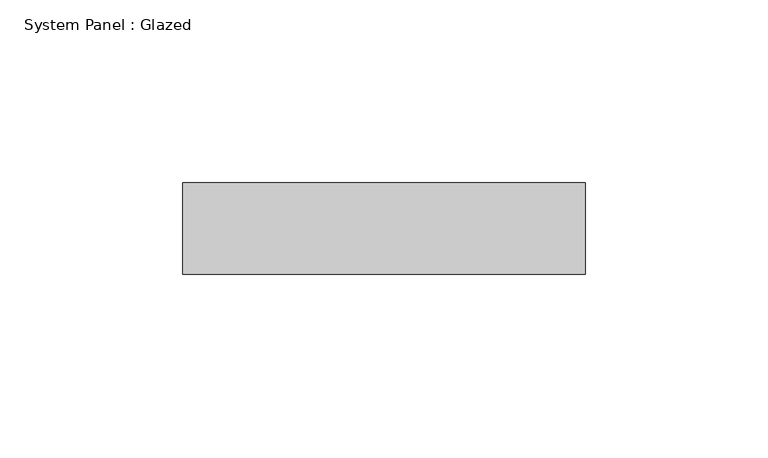
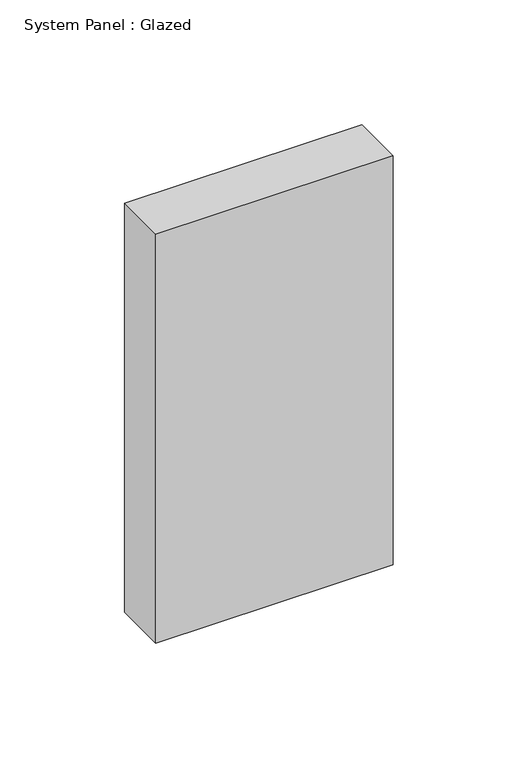
"""IFC4 building model written with IfcOpenShell, lengths in millimetres: plate geometry, System Panel : Glazed."""

from ifc_helpers import new_model, si_unit, origin, origin_with_axes, place, context, project, spatial, polyline, outline, extrude, source, transform, mapped, element, save


def system_panel_glazed_a6cffc9f(model_context):
    return source(origin(), model_context, "Body", "SweptSolid", [
        extrude(outline(polyline([(54.9468923, 24.5), (-54.9468923, 24.5), (-54.9468923, 49.5), (54.9468923, 49.5), (54.9468923, 24.5)])), origin_with_axes(), (0.0, 0.0, 1.0), 200.0),
    ])


if __name__ == "__main__":
    model = new_model("IFC4")
    model_context = context("Model", 3, world=origin())
    ifc_project = project(units=[si_unit("LENGTHUNIT", "METRE", prefix="MILLI")], contexts=[model_context])
    site = spatial("IfcSite", under=ifc_project)
    building = spatial("IfcBuilding", under=site)
    placement = place(None, origin())
    system_panel_glazed_shape = system_panel_glazed_a6cffc9f(model_context)
    element("IfcPlate", 1, ObjectType="System Panel : Glazed", at=placement, inside=building, context=model_context, shape_type="MappedRepresentation", body=[
        mapped(system_panel_glazed_shape, transform((0.0, 0.0, 0.0), x_axis=(1.0, 0.0, 0.0), y_axis=(0.0, 1.0, 0.0), z_axis=(0.0, 0.0, 1.0))),
    ])
    save(model, "model.ifc")

# Revit data of these elements
# Element 1 (IfcPlate, "System Panel : Glazed")
#   Materials on its faces: "Glass"
# Materials
#   "Glass": class "Glass", colour RGB 218 227 224, transparency 0.85, Description = "Soda Lime Glass", Cost = 0
